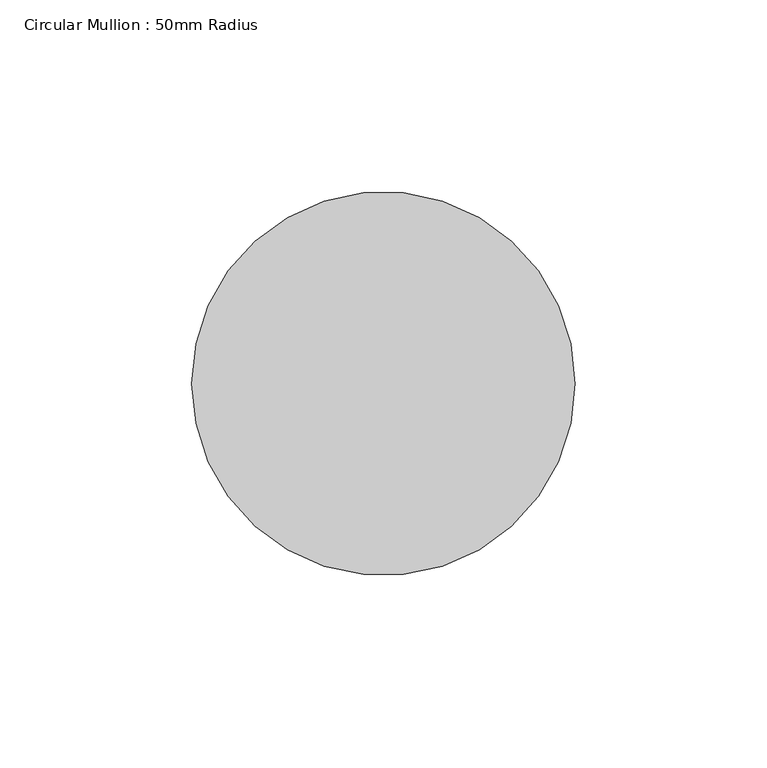
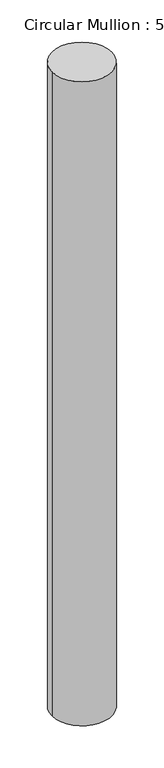
"""IFC4 building model written with IfcOpenShell, lengths in millimetres: member geometry, Circular Mullion : 50mm Radius."""

from ifc_helpers import new_model, si_unit, point, frame, origin, origin_2d, place, context, project, spatial, circle_curve, trimmed, segment, composite_curve, outline, extrude, source, transform, mapped, element, save


def circular_mullion_50mm_radius_4605ae1c(model_context):
    return source(origin(), model_context, "Body", "SweptSolid", [
        extrude(outline(composite_curve([segment(trimmed(circle_curve(origin_2d(), 50.0), [point((50.0, 0.0))], [point((-50.0, 0.0))], False, "CARTESIAN"), True, "CONTINUOUS"), segment(trimmed(circle_curve(origin_2d(), 50.0), [point((-50.0, 0.0))], [point((50.0, 0.0))], False, "CARTESIAN"), True, "CONTINUOUS")], self_intersect=False)), frame((0.0, 0.0, -1137.6830714), z_axis=(0.0, 0.0, 1.0), x_axis=(1.0, 0.0, 0.0)), (0.0, 0.0, 1.0), 1137.6830714),
    ])


if __name__ == "__main__":
    model = new_model("IFC4")
    model_context = context("Model", 3, world=origin())
    ifc_project = project(units=[si_unit("LENGTHUNIT", "METRE", prefix="MILLI")], contexts=[model_context])
    site = spatial("IfcSite", under=ifc_project)
    building = spatial("IfcBuilding", under=site)
    placement = place(None, origin())
    circular_mullion_50mm_radius_shape = circular_mullion_50mm_radius_4605ae1c(model_context)
    element("IfcMember", 1, ObjectType="Circular Mullion : 50mm Radius", at=placement, inside=building, context=model_context, shape_type="MappedRepresentation", body=[
        mapped(circular_mullion_50mm_radius_shape, transform((0.0, 0.0, 0.0), x_axis=(1.0, 0.0, 0.0), y_axis=(0.0, 1.0, 0.0), z_axis=(0.0, 0.0, 1.0))),
    ])
    save(model, "model.ifc")

# Revit data of these elements
# Type "Circular Mullion : 50mm Radius"
#   built-in parameter 1007350 = 0.164042 (stored number, unit not read)
# Element 1 (IfcMember, "Circular Mullion : 50mm Radius")
#   Materials on its faces: "Aluminium"
# Materials
#   "Aluminium": class "Metal", colour RGB 247 247 247, transparency 0, Description = "Aluminium 6061", Cost = 0
